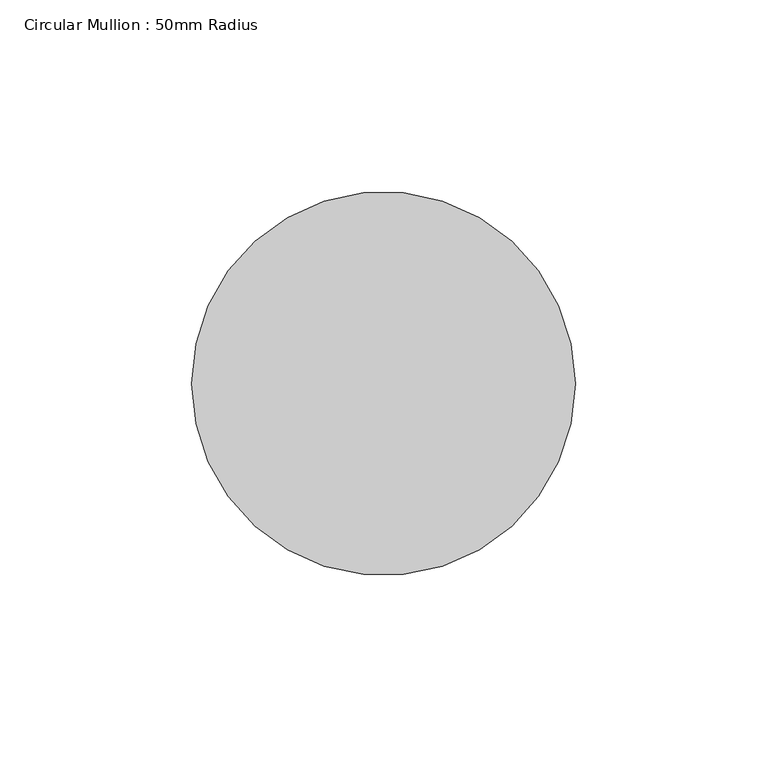
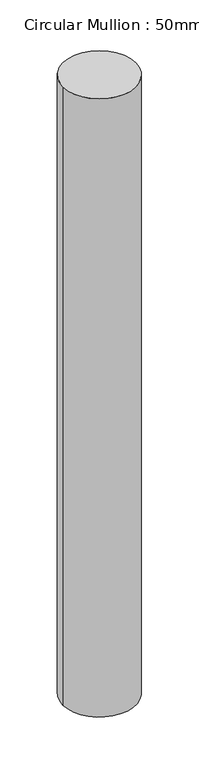
"""IFC4 building model written with IfcOpenShell, lengths in millimetres: member geometry, Circular Mullion : 50mm Radius."""

from ifc_helpers import new_model, si_unit, point, frame, origin, origin_2d, place, context, project, spatial, circle_curve, trimmed, segment, composite_curve, outline, extrude, source, transform, mapped, element, save


def circular_mullion_50mm_radius_93faa5ce(model_context):
    return source(origin(), model_context, "Body", "SweptSolid", [
        extrude(outline(composite_curve([segment(trimmed(circle_curve(origin_2d(), 50.0), [point((50.0, 0.0))], [point((-50.0, 0.0))], False, "CARTESIAN"), True, "CONTINUOUS"), segment(trimmed(circle_curve(origin_2d(), 50.0), [point((-50.0, 0.0))], [point((50.0, 0.0))], False, "CARTESIAN"), True, "CONTINUOUS")], self_intersect=False)), frame((0.0, 0.0, -898.6252925), z_axis=(0.0, 0.0, 1.0), x_axis=(1.0, 0.0, 0.0)), (0.0, 0.0, 1.0), 898.6252925),
    ])


if __name__ == "__main__":
    model = new_model("IFC4")
    model_context = context("Model", 3, world=origin())
    ifc_project = project(units=[si_unit("LENGTHUNIT", "METRE", prefix="MILLI")], contexts=[model_context])
    site = spatial("IfcSite", under=ifc_project)
    building = spatial("IfcBuilding", under=site)
    placement = place(None, origin())
    circular_mullion_50mm_radius_shape = circular_mullion_50mm_radius_93faa5ce(model_context)
    element("IfcMember", 1, ObjectType="Circular Mullion : 50mm Radius", at=placement, inside=building, context=model_context, shape_type="MappedRepresentation", body=[
        mapped(circular_mullion_50mm_radius_shape, transform((0.0, 0.0, 0.0), x_axis=(1.0, 0.0, 0.0), y_axis=(0.0, 1.0, 0.0), z_axis=(0.0, 0.0, 1.0))),
    ])
    save(model, "model.ifc")

# Revit data of these elements
# Type "Circular Mullion : 50mm Radius"
#   built-in parameter 1007350 = 0.164042 (stored number, unit not read)
# Element 1 (IfcMember, "Circular Mullion : 50mm Radius")
#   Materials on its faces: "Aluminium"
# Materials
#   "Aluminium": class "Metal", colour RGB 247 247 247, transparency 0, Description = "Aluminium 6061", Cost = 0
